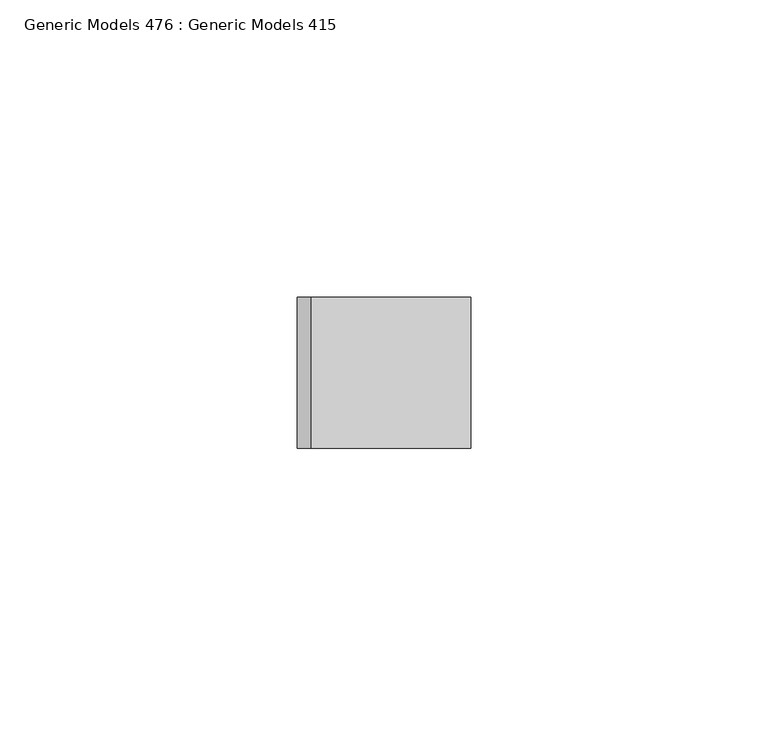
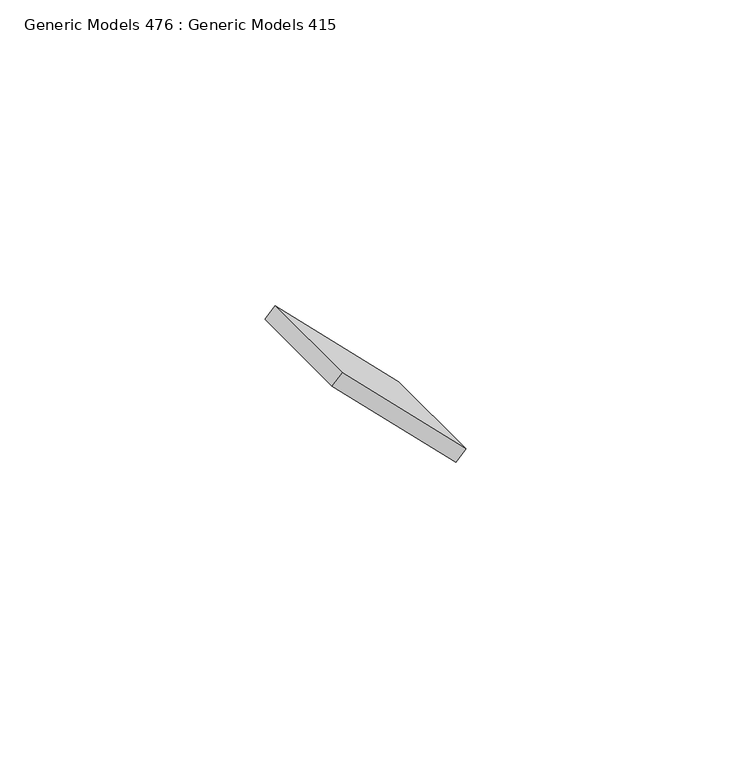
"""IFC4 building model written with IfcOpenShell, lengths in millimetres: proxy geometry, Generic Models 476 : Generic Models 415."""

import ifcopenshell
import ifcopenshell.guid

model = None  # the IFC model being written
_history = None  # IfcOwnerHistory: only IFC2X3 demands one
_inside = {}  # id of a spatial element -> (the spatial element, [elements in it])
_under = {}  # id of a project, library or spatial element -> (it, [spatial elements below it])
_declared = {}  # id of a project -> (the project, [libraries it declares])
_typed = {}  # id of a type object -> (the type object, [elements of that type])
_made_of = {}  # id of a material, layer set ... -> (it, [elements and type objects made of it])


def new_model(schema):
    """Start an empty IFC model of exactly this schema.

    Asked for "IFC4X3", IfcOpenShell would pick the latest addendum, in which some entities
    have other attributes; the version numbers below select the first issue.
    IFC2X3 requires an IfcOwnerHistory on every rooted entity: one is made here for all.
    """
    global model, _history
    if schema == "IFC4X3":
        model = ifcopenshell.file(schema_version=(4, 3, 0, 0))
    else:
        model = ifcopenshell.file(schema=schema)
    _inside.clear()
    _under.clear()
    _declared.clear()
    _typed.clear()
    _made_of.clear()
    _history = None
    if model.schema == "IFC2X3":
        org = make("IfcOrganization", Name="unknown")
        user = make(
            "IfcPersonAndOrganization",
            ThePerson=make("IfcPerson", FamilyName="unknown"),
            TheOrganization=org,
        )
        app = make(
            "IfcApplication",
            ApplicationDeveloper=org,
            Version="unknown",
            ApplicationFullName="unknown",
            ApplicationIdentifier="unknown",
        )
        _history = make(
            "IfcOwnerHistory",
            OwningUser=user,
            OwningApplication=app,
            ChangeAction="ADDED",
            CreationDate=0,
        )
    return model


def make(cls, **values):
    """One entity of the class cls with the attributes given. An attribute that is None is left unset."""
    return model.create_entity(
        cls, **{name: value for name, value in values.items() if value is not None}
    )


def rooted(cls, **values):
    """An entity with a GlobalId (a new one), such as an element, a storey or a relation."""
    return make(cls, GlobalId=ifcopenshell.guid.new(), OwnerHistory=_history, **values)


def si_unit(unit_type, name, prefix=None):
    """IfcSIUnit, for example si_unit("LENGTHUNIT", "METRE", prefix="MILLI")."""
    return make("IfcSIUnit", UnitType=unit_type, Prefix=prefix, Name=name)


def assignment(units):
    """IfcUnitAssignment: the units of a project."""
    return None if units is None else make("IfcUnitAssignment", Units=units)


def point(xyz):
    """IfcCartesianPoint."""
    return None if xyz is None else make("IfcCartesianPoint", Coordinates=xyz)


def direction(xyz):
    """IfcDirection."""
    return None if xyz is None else make("IfcDirection", DirectionRatios=xyz)


def frame(location, z_axis=None, x_axis=None):
    """IfcAxis2Placement3D, a coordinate frame: its origin and axes. An axis left out is left unset."""
    return make(
        "IfcAxis2Placement3D",
        Location=point(location),
        Axis=direction(z_axis),
        RefDirection=direction(x_axis),
    )


def origin():
    """The frame at (0, 0, 0) with its axes left unset."""
    return frame((0.0, 0.0, 0.0))


def place(relative_to, where):
    """IfcLocalPlacement: puts the frame where relative to a parent placement (None: the world)."""
    return make(
        "IfcLocalPlacement", PlacementRelTo=relative_to, RelativePlacement=where
    )


def context(
    kind, dimensions, precision=None, world=None, true_north=None, identifier=None
):
    """IfcGeometricRepresentationContext, for example the 3D "Model" context."""
    return make(
        "IfcGeometricRepresentationContext",
        ContextIdentifier=identifier,
        ContextType=kind,
        CoordinateSpaceDimension=dimensions,
        Precision=precision,
        WorldCoordinateSystem=world,
        TrueNorth=true_north,
    )


def project(units=None, contexts=None):
    """IfcProject with its units and contexts."""
    return rooted(
        "IfcProject",
        Name="project",
        RepresentationContexts=contexts,
        UnitsInContext=assignment(units),
    )


def spatial(cls, under=None, at=None, **own):
    """A site, building, storey or space (cls), placed at a placement, below another one or the project."""
    s = rooted(cls, ObjectPlacement=at, **own)
    if under is not None:
        _under.setdefault(under.id(), (under, []))[1].append(s)
    return s


def polyline(points):
    """IfcPolyline through the points."""
    return make("IfcPolyline", Points=[point(p) for p in points])


def outline(outer, holes=None, kind="AREA"):
    """IfcArbitraryClosedProfileDef: a profile drawn as a closed curve; with holes, ...WithVoids."""
    if holes is None:
        return make("IfcArbitraryClosedProfileDef", ProfileType=kind, OuterCurve=outer)
    return make(
        "IfcArbitraryProfileDefWithVoids",
        ProfileType=kind,
        OuterCurve=outer,
        InnerCurves=holes,
    )


def extrude(swept, where, along, depth):
    """IfcExtrudedAreaSolid: the profile swept, set in the frame where, extruded along a direction by depth."""
    return make(
        "IfcExtrudedAreaSolid",
        SweptArea=swept,
        Position=where,
        ExtrudedDirection=direction(along),
        Depth=depth,
    )


def shape(context_of_items, identifier, shape_type, items):
    """IfcShapeRepresentation: the items that make up one representation, for example the "Body"."""
    return make(
        "IfcShapeRepresentation",
        ContextOfItems=context_of_items,
        RepresentationIdentifier=identifier,
        RepresentationType=shape_type,
        Items=items,
    )


def source(mapping_origin, context_of_items, identifier, shape_type, items):
    """IfcRepresentationMap: a shape defined once, which mapped items show again and again."""
    return make(
        "IfcRepresentationMap",
        MappingOrigin=mapping_origin,
        MappedRepresentation=shape(context_of_items, identifier, shape_type, items),
    )


def transform(
    local_origin,
    x_axis=None,
    y_axis=None,
    z_axis=None,
    scale=None,
    scale2=None,
    scale3=None,
    uniform=True,
):
    """IfcCartesianTransformationOperator3D, or its non-uniform kind. x_axis, y_axis, z_axis: its Axis1, 2, 3."""
    if uniform:
        return make(
            "IfcCartesianTransformationOperator3D",
            Axis1=direction(x_axis),
            Axis2=direction(y_axis),
            LocalOrigin=point(local_origin),
            Scale=scale,
            Axis3=direction(z_axis),
        )
    return make(
        "IfcCartesianTransformationOperator3DnonUniform",
        Axis1=direction(x_axis),
        Axis2=direction(y_axis),
        LocalOrigin=point(local_origin),
        Scale=scale,
        Axis3=direction(z_axis),
        Scale2=scale2,
        Scale3=scale3,
    )


def mapped(mapping_source, mapping_target):
    """IfcMappedItem: shows the shape of a source again, moved by a transform."""
    return make(
        "IfcMappedItem", MappingSource=mapping_source, MappingTarget=mapping_target
    )


def made_of(thing, what):
    """Note that an element or type object is made of a material, layer set ...; save() writes the relation."""
    if what is not None:
        _made_of.setdefault(what.id(), (what, []))[1].append(thing)
    return thing


def element(
    cls,
    number,
    at=None,
    inside=None,
    cuts=None,
    type_object=None,
    material=None,
    context=None,
    identifier="Body",
    shape_type=None,
    held_by="IfcProductDefinitionShape",
    body=None,
    shapes=None,
    **own,
):
    """One element of the class cls, such as IfcWall. Its Tag is "e" and its number.

    at: its placement. inside: the storey or other place that contains it. cuts: it is an
    opening in that element (IfcRelVoidsElement). A single representation is given by context,
    identifier, shape_type and body (its items); several are given by shapes. held_by: the class
    of the entity that holds the representations. save() writes the other relations.
    """
    e = rooted(cls, Tag="e%d" % number, ObjectPlacement=at, **own)
    if body is not None:
        shapes = [shape(context, identifier, shape_type, body)]
    if shapes is not None:
        e.Representation = make(held_by, Representations=shapes)
    if inside is not None:
        _inside.setdefault(inside.id(), (inside, []))[1].append(e)
    if cuts is not None:
        rooted(
            "IfcRelVoidsElement", RelatingBuildingElement=cuts, RelatedOpeningElement=e
        )
    if type_object is not None:
        _typed.setdefault(type_object.id(), (type_object, []))[1].append(e)
    return made_of(e, material)


def aggregate(whole, parts):
    """IfcRelAggregates: a whole, such as a stair, and the parts it consists of."""
    return rooted("IfcRelAggregates", RelatingObject=whole, RelatedObjects=parts)


def save(model, path):
    """Write the relations noted so far, then the file.

    IfcRelAggregates (storeys below a building ...), IfcRelContainedInSpatialStructure (elements
    in a storey), IfcRelDefinesByType, IfcRelAssociatesMaterial and IfcRelDeclares: one each for
    every whole, place, type object, material and project.
    """
    for whole, parts in _under.values():
        aggregate(whole, parts)
    for where, things in _inside.values():
        rooted(
            "IfcRelContainedInSpatialStructure",
            RelatedElements=things,
            RelatingStructure=where,
        )
    for kind, things in _typed.values():
        rooted("IfcRelDefinesByType", RelatedObjects=things, RelatingType=kind)
    for what, things in _made_of.values():
        rooted("IfcRelAssociatesMaterial", RelatedObjects=things, RelatingMaterial=what)
    for by, libraries in _declared.values():
        rooted("IfcRelDeclares", RelatingContext=by, RelatedDefinitions=libraries)
    model.write(path)


def generic_models_476_generic_models_415_39bddc49(model_context):
    return source(origin(), model_context, "Body", "SweptSolid", [
        extrude(outline(polyline([(0.0, -38.1), (0.0, 0.0), (25.4, 0.0), (25.4, -38.1), (0.0, -38.1)])), frame((-6869.8996186, -4475.9863946, 127972.0002957), z_axis=(0.7071067811864907, 0.0, 0.7071067811866044), x_axis=(0.0, -1.0, 0.0)), (0.0, 0.0, 1.0), 3.175),
    ])


if __name__ == "__main__":
    model = new_model("IFC4")
    model_context = context("Model", 3, world=origin())
    ifc_project = project(units=[si_unit("LENGTHUNIT", "METRE", prefix="MILLI")], contexts=[model_context])
    site = spatial("IfcSite", under=ifc_project)
    building = spatial("IfcBuilding", under=site)
    placement = place(None, origin())
    generic_models_476_generic_models_415_shape = generic_models_476_generic_models_415_39bddc49(model_context)
    element("IfcBuildingElementProxy", 1, Name="Generic Models 476 : Generic Models 415", ObjectType="Generic Models 476 : Generic Models 415", at=placement, inside=building, context=model_context, shape_type="MappedRepresentation", body=[
        mapped(generic_models_476_generic_models_415_shape, transform((0.0, 0.0, 0.0), x_axis=(1.0, 0.0, 0.0), y_axis=(0.0, 1.0, 0.0), z_axis=(0.0, 0.0, 1.0))),
    ])
    save(model, "model.ifc")

# Revit data of these elements
# Element 1 (IfcBuildingElementProxy, "Generic Models 476 : Generic Models 415")
#   Materials on its faces: "_WELDED STEEL TABS FOR LOUVER ATTACHMENT"
# Materials
#   "_WELDED STEEL TABS FOR LOUVER ATTACHMENT": class "Metal", colour RGB 199 199 199, transparency 0, Description = "Structural steel 50ksi", Cost = 0
